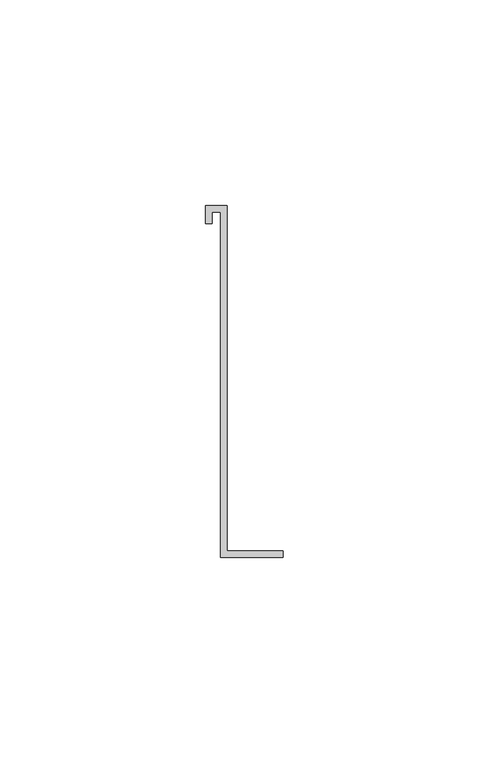
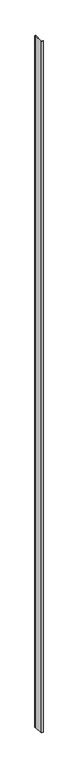
"""IFC4 building model written with IfcOpenShell, lengths in millimetres: proxy geometry, Generic Models 7:Generic Models 1:3:Generic Models 1:3 : Generic Models 7:Generic Models 1:305549:3:Generic Models 1:3:Generic Models 1:3 : Generic Models 7:Generic Models 1:305549:3 : Generic Models 7:Generic Models 1:3:Generic Models 1:3 : Generic Models 7:Generic Models 1:305549:301244:15 : Generic Models 7:Generic Models 1:3:Generic Models 1:3 : Generic Models 7:Generic Models 1:305549:3:Generic Models 1:3:Generic Models 1:3 : Generic Models 7:Generic Models 1:305549:3 : Generic Models 7:Generic Models 1:3:Generic Models 1:3 : Generic Models 7:Generic Models 1:305549:301244:308848."""

from ifc_helpers import new_model, si_unit, frame, origin, place, context, project, spatial, polyline, outline, extrude, source, transform, mapped, element, save


def generic_models_cf2e6ea0(model_context):
    return source(origin(), model_context, "Body", "SweptSolid", [
        extrude(outline(polyline([(667607.9581314, -568252.7471585), (667607.9581314, -568168.7805453), (667605.8617598, -568168.7805453), (667605.8617598, -568171.5803719), (667604.2742598, -568171.5803719), (667604.2742598, -568167.1930453), (667609.5456314, -568167.1930453), (667609.5456314, -568251.1596585), (667623.1314112, -568251.1596585), (667623.1314112, -568252.7471585), (667607.9581314, -568252.7471585)])), frame((0.0, 0.0, 50.8), z_axis=(0.0, 0.0, 1.0), x_axis=(1.0, 0.0, 0.0)), (0.0, 0.0, 1.0), 6115.7954438),
    ])


if __name__ == "__main__":
    model = new_model("IFC4")
    model_context = context("Model", 3, world=origin())
    ifc_project = project(units=[si_unit("LENGTHUNIT", "METRE", prefix="MILLI")], contexts=[model_context])
    site = spatial("IfcSite", under=ifc_project)
    building = spatial("IfcBuilding", under=site)
    placement = place(None, origin())
    generic_models_shape = generic_models_cf2e6ea0(model_context)
    element("IfcBuildingElementProxy", 1, Name="Generic Models 7:Generic Models 1:3:Generic Models 1:3 : Generic Models 7:Generic Models 1:305549:3:Generic Models 1:3:Generic Models 1:3 : Generic Models 7:Generic Models 1:305549:3 : Generic Models 7:Generic Models 1:3:Generic Models 1:3 : Generic Models 7:Generic Models 1:305549:301244:15 : Generic Models 7:Generic Models 1:3:Generic Models 1:3 : Generic Models 7:Generic Models 1:305549:3:Generic Models 1:3:Generic Models 1:3 : Generic Models 7:Generic Models 1:305549:3 : Generic Models 7:Generic Models 1:3:Generic Models 1:3 : Generic Models 7:Generic Models 1:305549:301244:308848", ObjectType="Generic Models 7:Generic Models 1:3:Generic Models 1:3 : Generic Models 7:Generic Models 1:305549:3:Generic Models 1:3:Generic Models 1:3 : Generic Models 7:Generic Models 1:305549:3 : Generic Models 7:Generic Models 1:3:Generic Models 1:3 : Generic Models 7:Generic Models 1:305549:301244:15 : Generic Models 7:Generic Models 1:3:Generic Models 1:3 : Generic Models 7:Generic Models 1:305549:3:Generic Models 1:3:Generic Models 1:3 : Generic Models 7:Generic Models 1:305549:3 : Generic Models 7:Generic Models 1:3:Generic Models 1:3 : Generic Models 7:Generic Models 1:305549:301244:308848", at=placement, inside=building, context=model_context, shape_type="MappedRepresentation", body=[
        mapped(generic_models_shape, transform((0.0, 0.0, 0.0), x_axis=(1.0, 0.0, 0.0), y_axis=(0.0, 1.0, 0.0), z_axis=(0.0, 0.0, 1.0))),
    ])
    save(model, "model.ifc")

# Revit data of these elements
# Type "Generic Models 7:Generic Models 1:3:Generic Models 1:3 : Generic Models 7:Generic Models 1:305549:3:Generic Models 1:3:Generic Models 1:3 : Generic Models 7:Generic Models 1:305549:3 : Generic Models 7:Generic Models 1:3:Generic Models 1:3 : Generic Models 7:Generic Models 1:305549:301244:15 : Generic Models 7:Generic Models 1:3:Generic Models 1:3 : Generic Models 7:Generic Models 1:305549:3:Generic Models 1:3:Generic Models 1:3 : Generic Models 7:Generic Models 1:305549:3 : Generic Models 7:Generic Models 1:3:Generic Models 1:3 : Generic Models 7:Generic Models 1:305549:301244:308848"
#   NameOverride = "Generic Models 7:Generic Models 1:3:Generic Models 1:3 : Generic Models 7:Generic Models 1:305549:3:Generic Models 1:3:Generic Models 1:3 : Generic Models 7:Generic Models 1:305549:3 : Generic Models 7:Generic Models 1:3:Generic Models 1:3 : Generic Models 7:Generic Models 1:305549:301244:308848"
#   ObjectTypeOverride = "Generic Models 1:3:Generic Models 1:3 : Generic Models 7:Generic Models 1:305549:3 : Generic Models 7:Generic Models 1:3:Generic Models 1:3 : Generic Models 7:Generic Models 1:305549:301244"
#   Reference = "Generic Models 1"
#   Tag = "308848"
# Element 1 (IfcBuildingElementProxy, "Generic Models 7:Generic Models 1:3:Generic Models 1:3 : Generic Models 7:Generic Models 1:305549:3:Generic Models 1:3:Generic Models 1:3 : Generic Models 7:Generic Models 1:305549:3 : Generic Models 7:Generic Models 1:3:Generic Models 1:3 : Generic Models 7:Generic Models 1:305549:301244:15 : Generic Models 7:Generic Models 1:3:Generic Models 1:3 : Generic Models 7:Generic Models 1:305549:3:Generic Models 1:3:Generic Models 1:3 : Generic Models 7:Generic Models 1:305549:3 : Generic Models 7:Generic Models 1:3:Generic Models 1:3 : Generic Models 7:Generic Models 1:305549:301244:308848")
#   Materials on its faces: "BRAKE METAL CLOSURE TRIM"
# Materials
#   "BRAKE METAL CLOSURE TRIM": class "Unassigned", colour RGB 182 182 182, transparency 0, Cost = 0
